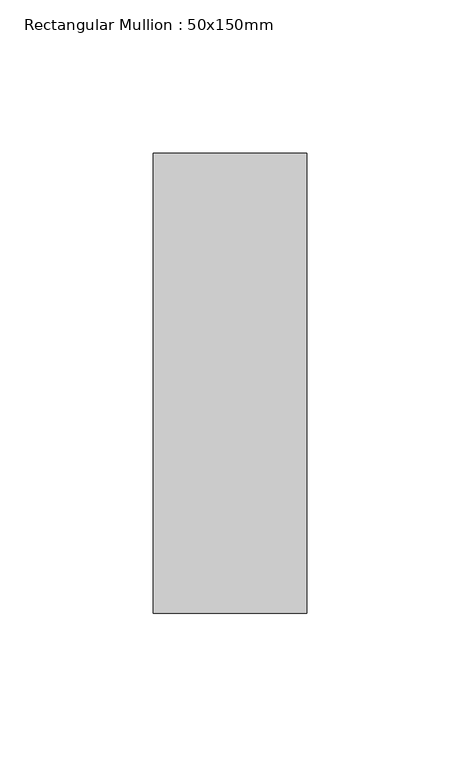
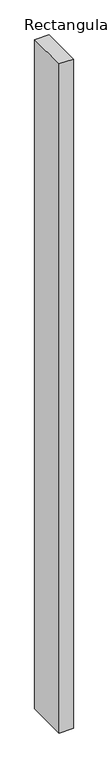
"""IFC4 building model written with IfcOpenShell, lengths in millimetres: member geometry, Rectangular Mullion : 50x150mm."""

from ifc_helpers import new_model, si_unit, frame, origin, place, context, project, spatial, polyline, outline, extrude, source, transform, mapped, element, save


def rectangular_mullion_50x150mm_eb9201c3(model_context):
    return source(origin(), model_context, "Body", "SweptSolid", [
        extrude(outline(polyline([(25.0, 75.0), (25.0, -75.0), (-25.0, -75.0), (-25.0, 75.0), (25.0, 75.0)])), frame((0.0, 0.0, -2500.0), z_axis=(0.0, 0.0, 1.0), x_axis=(1.0, 0.0, 0.0)), (0.0, 0.0, 1.0), 2500.0),
    ])


if __name__ == "__main__":
    model = new_model("IFC4")
    model_context = context("Model", 3, world=origin())
    ifc_project = project(units=[si_unit("LENGTHUNIT", "METRE", prefix="MILLI")], contexts=[model_context])
    site = spatial("IfcSite", under=ifc_project)
    building = spatial("IfcBuilding", under=site)
    placement = place(None, origin())
    rectangular_mullion_50x150mm_shape = rectangular_mullion_50x150mm_eb9201c3(model_context)
    element("IfcMember", 1, ObjectType="Rectangular Mullion : 50x150mm", at=placement, inside=building, context=model_context, shape_type="MappedRepresentation", body=[
        mapped(rectangular_mullion_50x150mm_shape, transform((0.0, 0.0, 0.0), x_axis=(1.0, 0.0, 0.0), y_axis=(0.0, 1.0, 0.0), z_axis=(0.0, 0.0, 1.0))),
    ])
    save(model, "model.ifc")

# Revit data of these elements
# Type "Rectangular Mullion : 50x150mm"
#   Keynote = "H11"
#   built-in parameter 1007304 = 0.492126 (stored number, unit not read)
#   built-in parameter 1007301 = 0.082021 (stored number, unit not read)
#   built-in parameter 1007300 = 0.082021 (stored number, unit not read)
# Element 1 (IfcMember, "Rectangular Mullion : 50x150mm")
#   Materials on its faces: "Aluminium"
# Materials
#   "Aluminium": class "Metal", colour RGB 247 247 247, transparency 0, Description = "Aluminium 6061", Cost = 0
